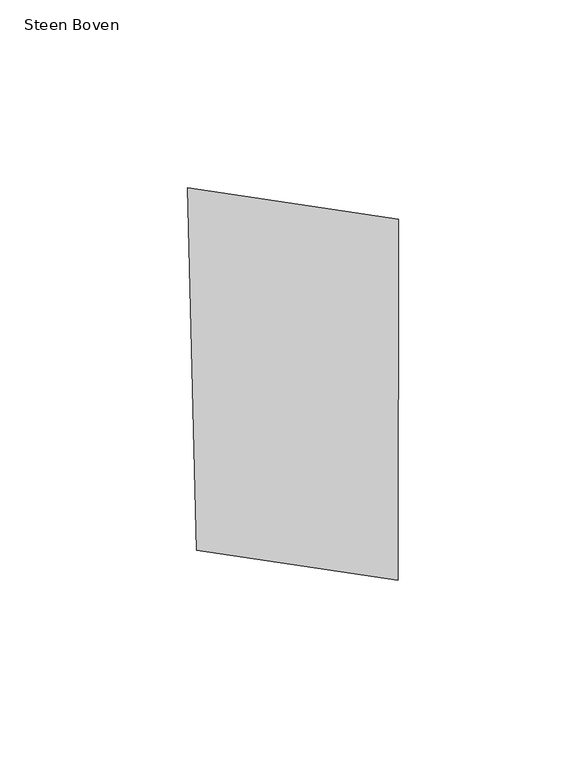
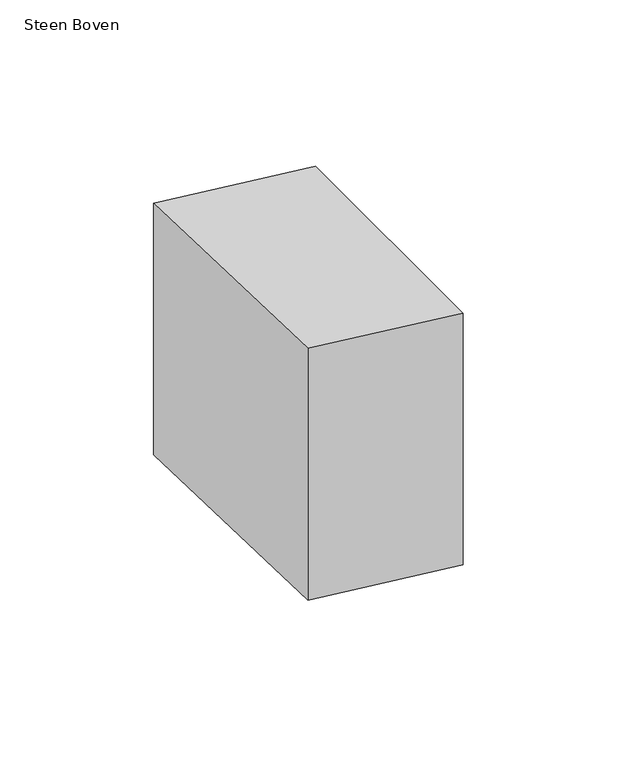
"""IFC4 building model written with IfcOpenShell, lengths in millimetres: proxy geometry, 00_GMA_steen_versie_4 : Steen Boven."""

from ifc_helpers import new_model, si_unit, origin, origin_with_axes, place, context, project, spatial, polyline, outline, extrude, source, transform, mapped, element, save


def steen_boven_d8d8c79b(model_context):
    return source(origin(), model_context, "Body", "SweptSolid", [
        extrude(outline(polyline([(100.6605952, 119.86202), (100.5581516, 23.7906576), (47.0085955, 31.6852786), (44.6025305, 128.1448028), (100.6605952, 119.86202)])), origin_with_axes(), (0.0, 0.0, 1.0), 100.0),
    ])


if __name__ == "__main__":
    model = new_model("IFC4")
    model_context = context("Model", 3, world=origin())
    ifc_project = project(units=[si_unit("LENGTHUNIT", "METRE", prefix="MILLI")], contexts=[model_context])
    site = spatial("IfcSite", under=ifc_project)
    building = spatial("IfcBuilding", under=site)
    placement = place(None, origin())
    steen_boven_shape = steen_boven_d8d8c79b(model_context)
    element("IfcBuildingElementProxy", 1, Name="00_GMA_steen_versie_4 : Steen Boven", ObjectType="00_GMA_steen_versie_4 : Steen Boven", at=placement, inside=building, context=model_context, shape_type="MappedRepresentation", body=[
        mapped(steen_boven_shape, transform((0.0, 0.0, 0.0), x_axis=(1.0, 0.0, 0.0), y_axis=(0.0, 1.0, 0.0), z_axis=(0.0, 0.0, 1.0))),
    ])
    save(model, "model.ifc")

# Revit data of these elements
# Type "00_GMA_steen_versie_4 : Steen Boven"
#   StootVoegHalfBoven [instance default] = 5 mm
#   StootVoegHalf [instance default] = 5 mm
#   StootVoegBreedteOnder = 10 mm
#   StootVoegBreedteBoven = 10 mm
#   Steendikte = 100 mm
#   LintVoegOnderHalf = 5 mm
#   LintVoegOnder = 10 mm
#   LintVoegBovenHalf = 0 mm
#   LintVoegBoven = 0 mm
#   materiaal = none
#   MateriaalVoeg = none
#   Default Elevation = 0
